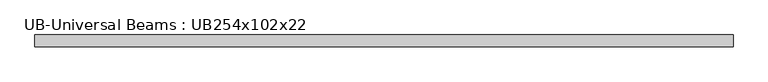
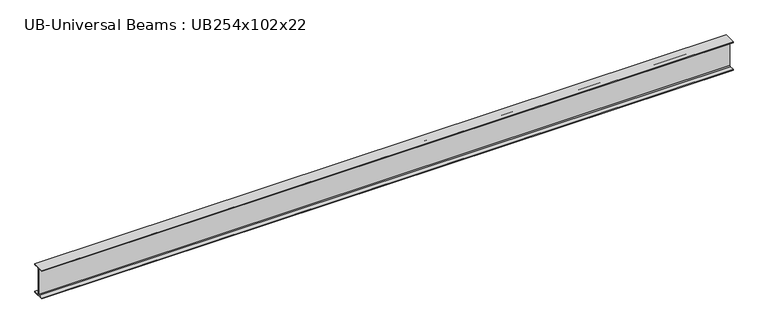
"""IFC4 building model written with IfcOpenShell, lengths in millimetres: beam geometry, UB-Universal Beams : UB254x102x22."""

from ifc_helpers import new_model, si_unit, point, frame, frame_2d, origin, place, context, project, spatial, polyline, circle_curve, trimmed, segment, composite_curve, outline, extrude, source, transform, mapped, element, save


def ub_universal_beams_ub254x102x22_dcacaae8(model_context):
    return source(origin(), model_context, "Body", "SweptSolid", [
        extrude(outline(composite_curve([segment(polyline([(50.8, -120.2), (50.8, -127.0), (-50.8, -127.0), (-50.8, -120.2), (-10.45, -120.2)]), True, "CONTINUOUS"), segment(trimmed(circle_curve(frame_2d((-10.45, -112.6)), 7.6), [point((-10.45, -120.2))], [point((-2.85, -112.6))], True, "CARTESIAN"), True, "CONTINUOUS"), segment(polyline([(-2.85, -112.6), (-2.85, 112.6)]), True, "CONTINUOUS"), segment(trimmed(circle_curve(frame_2d((-10.45, 112.6)), 7.6), [point((-2.85, 112.6))], [point((-10.45, 120.2))], True, "CARTESIAN"), True, "CONTINUOUS"), segment(polyline([(-10.45, 120.2), (-50.8, 120.2), (-50.8, 127.0), (50.8, 127.0), (50.8, 120.2), (10.45, 120.2)]), True, "CONTINUOUS"), segment(trimmed(circle_curve(frame_2d((10.45, 112.6)), 7.6), [point((10.45, 120.2))], [point((2.85, 112.6))], True, "CARTESIAN"), True, "CONTINUOUS"), segment(polyline([(2.85, 112.6), (2.85, -112.6)]), True, "CONTINUOUS"), segment(trimmed(circle_curve(frame_2d((10.45, -112.6)), 7.6), [point((2.85, -112.6))], [point((10.45, -120.2))], True, "CARTESIAN"), True, "CONTINUOUS"), segment(polyline([(10.45, -120.2), (50.8, -120.2)]), True, "CONTINUOUS")], self_intersect=False)), frame((-2936.5, 0.0, 0.0), z_axis=(1.0, 0.0, 0.0), x_axis=(0.0, 1.0, 0.0)), (0.0, 0.0, 1.0), 5873.0),
    ])


if __name__ == "__main__":
    model = new_model("IFC4")
    model_context = context("Model", 3, world=origin())
    ifc_project = project(units=[si_unit("LENGTHUNIT", "METRE", prefix="MILLI")], contexts=[model_context])
    site = spatial("IfcSite", under=ifc_project)
    building = spatial("IfcBuilding", under=site)
    placement = place(None, origin())
    ub_universal_beams_ub254x102x22_shape = ub_universal_beams_ub254x102x22_dcacaae8(model_context)
    element("IfcBeam", 1, ObjectType="UB-Universal Beams : UB254x102x22", at=placement, inside=building, context=model_context, shape_type="MappedRepresentation", body=[
        mapped(ub_universal_beams_ub254x102x22_shape, transform((0.0, 0.0, 0.0), x_axis=(1.0, 0.0, 0.0), y_axis=(0.0, 1.0, 0.0), z_axis=(0.0, 0.0, 1.0))),
    ])
    save(model, "model.ifc")

# Revit data of these elements
# Type "UB-Universal Beams : UB254x102x22"
#   Section Name Key = "UB254X102X22"
#   Width = 10.16 cm
#   Web Thickness = 0.57 cm
#   Web Fillet = 0.76 cm
#   Warping Constant = 18200.0 cm⁶
#   Torsional Moment of Inertia = 4.15 cm⁴
#   Section Area = 28.0 cm²
#   Plastic Modulus weak axis = 37.3 cm³
#   Plastic Modulus strong axis = 259.0 cm³
#   Nominal Weight = 22.00 kgf/m
#   Moment of Inertia weak axis = 119.00 cm⁴
#   Moment of Inertia strong axis = 2841.00 cm⁴
#   Height = 25.4 cm
#   Flange Thickness = 0.68 cm
#   Elastic Modulus weak axis = 23.5 cm³
#   Elastic Modulus strong axis = 224.0 cm³
#   Centroid Vertical = 12.7 cm
#   Centroid Horizontal = 5.08 cm
#   Bolt Spacing = 5.4 cm
#   Length [instance default] = 1500 mm
#   Structural Material [instance default] = Metal - Steel 43-275
#   Type Comments = ""
#   Assembly Code = ""
# Element 1 (IfcBeam, "UB-Universal Beams : UB254x102x22")
#   Materials on its faces: "Metal - Steel 43-275"
# Materials
#   "Metal - Steel 43-275": class "Metal", colour RGB 247 247 247, transparency 0, Cost = 0
